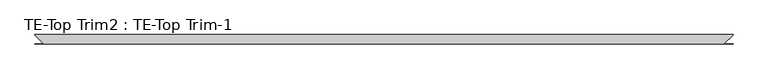
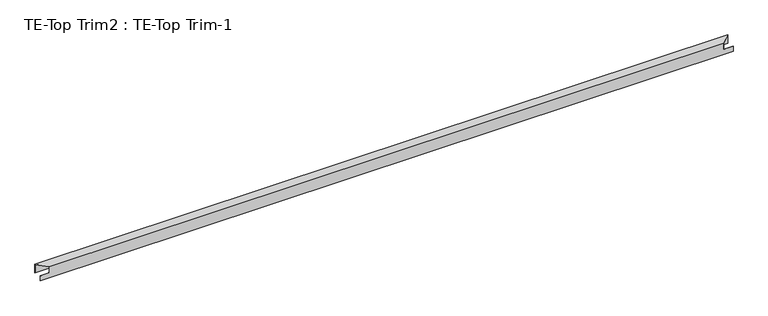
"""IFC4 building model written with IfcOpenShell, lengths in millimetres: proxy geometry, TE-Top Trim2 : TE-Top Trim-1."""

from ifc_helpers import new_model, si_unit, origin, place, context, project, spatial, faceted_brep, source, transform, mapped, element, save


def te_top_trim2_te_top_trim_1_ce3f5671(model_context):
    return source(origin(), model_context, "Body", "Brep", [
        faceted_brep([(587327.7934739, -531640.1093528, 2387.6), (587327.7934739, -531641.0023216, 2387.6), (587327.7934739, -531641.0023216, 2411.4125), (587327.7934739, -531640.1093528, 2411.4125), (587327.7934739, -531599.3917241, 2439.2929688), (587327.7934739, -531599.3917241, 2400.3), (587327.7934739, -531600.3289841, 2400.3), (587327.7934739, -531600.3289841, 2438.4), (587327.7934739, -531601.1251169, 2438.4), (587327.7934739, -531601.1251169, 2439.2929688), (590392.4558739, -531600.3289841, 2400.3), (590392.4558739, -531599.3917241, 2400.3), (590392.4558739, -531599.3917241, 2439.2929688), (590392.4558739, -531600.3190424, 2439.2929688), (590392.4558739, -531600.3190424, 2438.4), (590392.4558739, -531600.3289841, 2411.4125), (590392.4558739, -531641.0023216, 2387.6), (590392.4558739, -531640.1093528, 2387.6), (590392.4558739, -531640.1093528, 2411.4125), (590392.4558739, -531641.0023216, 2411.4125), (590351.7725947, -531641.0023216, 2411.4125), (590351.7725947, -531641.0023216, 2439.2929688), (587367.6706786, -531641.0023216, 2439.2929688), (587367.6706786, -531641.0023216, 2411.4125), (590352.6655635, -531640.1093528, 2438.4), (587366.7777099, -531640.1093528, 2438.4), (587366.7777099, -531640.1093528, 2411.4125), (590352.6655635, -531640.1093528, 2411.4125)], [[[0, 1, 2, 3]], [[4, 5, 6, 7, 8, 9]], [[10, 11, 12, 13, 14, 15]], [[16, 17, 18, 19]], [[1, 0, 17, 16]], [[1, 16, 19, 20, 21, 22, 23, 2]], [[12, 4, 9, 22, 21, 13]], [[5, 4, 12, 11]], [[6, 5, 11, 10]], [[7, 6, 10, 15, 14]], [[7, 14, 24, 25, 8]], [[17, 0, 3, 26, 25, 24, 27, 18]], [[27, 20, 19, 18]], [[20, 27, 24, 14, 13, 21]], [[23, 26, 3, 2]], [[26, 23, 22, 9, 8, 25]]]),
    ])


if __name__ == "__main__":
    model = new_model("IFC4")
    model_context = context("Model", 3, world=origin())
    ifc_project = project(units=[si_unit("LENGTHUNIT", "METRE", prefix="MILLI")], contexts=[model_context])
    site = spatial("IfcSite", under=ifc_project)
    building = spatial("IfcBuilding", under=site)
    placement = place(None, origin())
    te_top_trim2_te_top_trim_1_shape = te_top_trim2_te_top_trim_1_ce3f5671(model_context)
    element("IfcBuildingElementProxy", 1, Name="TE-Top Trim2 : TE-Top Trim-1", ObjectType="TE-Top Trim2 : TE-Top Trim-1", at=placement, inside=building, context=model_context, shape_type="MappedRepresentation", body=[
        mapped(te_top_trim2_te_top_trim_1_shape, transform((0.0, 0.0, 0.0), x_axis=(1.0, 0.0, 0.0), y_axis=(0.0, 1.0, 0.0), z_axis=(0.0, 0.0, 1.0))),
    ])
    save(model, "model.ifc")

# Revit data of these elements
# Element 1 (IfcBuildingElementProxy, "TE-Top Trim2 : TE-Top Trim-1")
#   Materials on its faces: "EDGE TRIM BY MTL PANEL MFR."
# Materials
#   "EDGE TRIM BY MTL PANEL MFR.": class "Generic", colour RGB 239 242 240, transparency 0, Cost = 0
